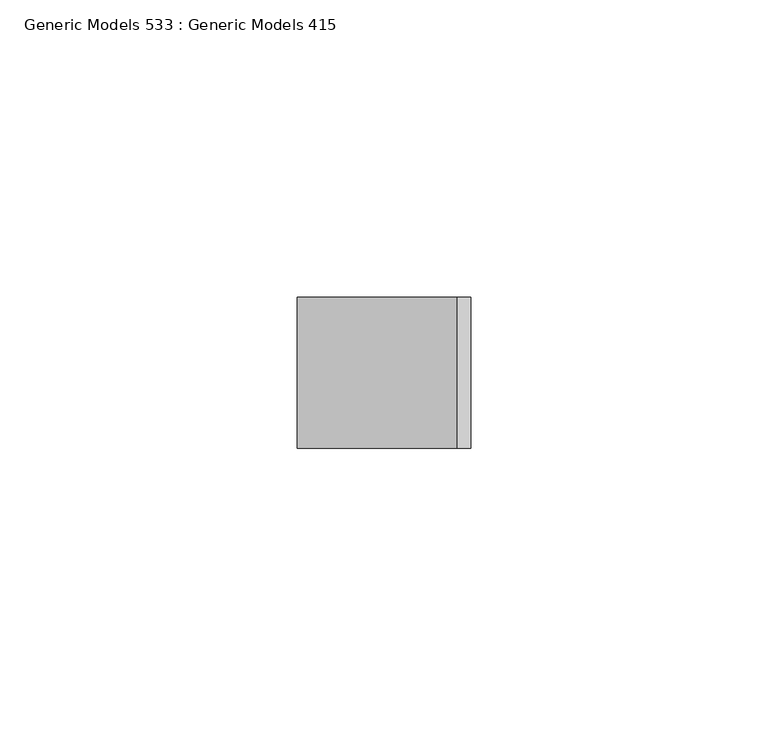
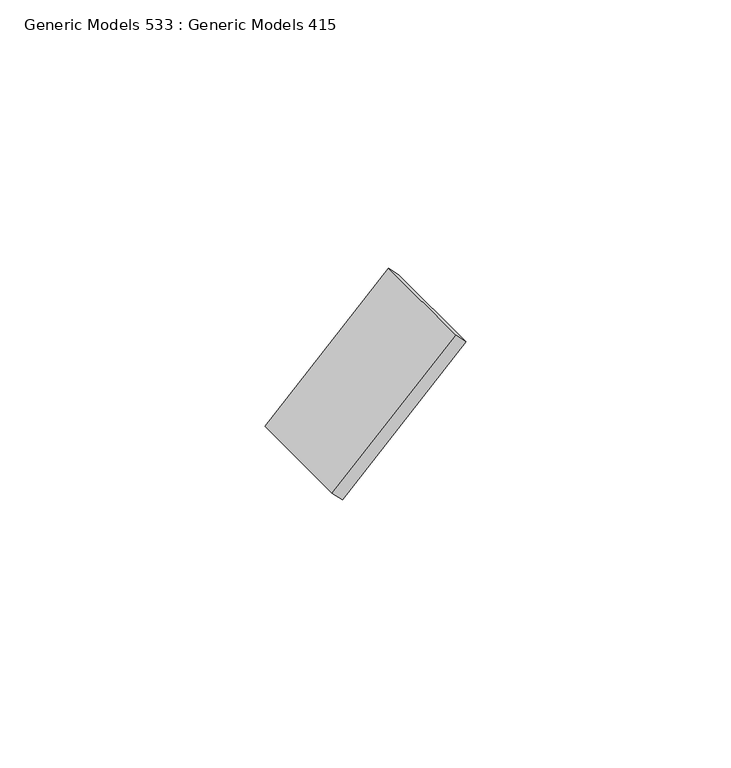
"""IFC4 building model written with IfcOpenShell, lengths in millimetres: proxy geometry, Generic Models 533 : Generic Models 415."""

import ifcopenshell
import ifcopenshell.guid

model = None  # the IFC model being written
_history = None  # IfcOwnerHistory: only IFC2X3 demands one
_inside = {}  # id of a spatial element -> (the spatial element, [elements in it])
_under = {}  # id of a project, library or spatial element -> (it, [spatial elements below it])
_declared = {}  # id of a project -> (the project, [libraries it declares])
_typed = {}  # id of a type object -> (the type object, [elements of that type])
_made_of = {}  # id of a material, layer set ... -> (it, [elements and type objects made of it])


def new_model(schema):
    """Start an empty IFC model of exactly this schema.

    Asked for "IFC4X3", IfcOpenShell would pick the latest addendum, in which some entities
    have other attributes; the version numbers below select the first issue.
    IFC2X3 requires an IfcOwnerHistory on every rooted entity: one is made here for all.
    """
    global model, _history
    if schema == "IFC4X3":
        model = ifcopenshell.file(schema_version=(4, 3, 0, 0))
    else:
        model = ifcopenshell.file(schema=schema)
    _inside.clear()
    _under.clear()
    _declared.clear()
    _typed.clear()
    _made_of.clear()
    _history = None
    if model.schema == "IFC2X3":
        org = make("IfcOrganization", Name="unknown")
        user = make(
            "IfcPersonAndOrganization",
            ThePerson=make("IfcPerson", FamilyName="unknown"),
            TheOrganization=org,
        )
        app = make(
            "IfcApplication",
            ApplicationDeveloper=org,
            Version="unknown",
            ApplicationFullName="unknown",
            ApplicationIdentifier="unknown",
        )
        _history = make(
            "IfcOwnerHistory",
            OwningUser=user,
            OwningApplication=app,
            ChangeAction="ADDED",
            CreationDate=0,
        )
    return model


def make(cls, **values):
    """One entity of the class cls with the attributes given. An attribute that is None is left unset."""
    return model.create_entity(
        cls, **{name: value for name, value in values.items() if value is not None}
    )


def rooted(cls, **values):
    """An entity with a GlobalId (a new one), such as an element, a storey or a relation."""
    return make(cls, GlobalId=ifcopenshell.guid.new(), OwnerHistory=_history, **values)


def si_unit(unit_type, name, prefix=None):
    """IfcSIUnit, for example si_unit("LENGTHUNIT", "METRE", prefix="MILLI")."""
    return make("IfcSIUnit", UnitType=unit_type, Prefix=prefix, Name=name)


def assignment(units):
    """IfcUnitAssignment: the units of a project."""
    return None if units is None else make("IfcUnitAssignment", Units=units)


def point(xyz):
    """IfcCartesianPoint."""
    return None if xyz is None else make("IfcCartesianPoint", Coordinates=xyz)


def direction(xyz):
    """IfcDirection."""
    return None if xyz is None else make("IfcDirection", DirectionRatios=xyz)


def frame(location, z_axis=None, x_axis=None):
    """IfcAxis2Placement3D, a coordinate frame: its origin and axes. An axis left out is left unset."""
    return make(
        "IfcAxis2Placement3D",
        Location=point(location),
        Axis=direction(z_axis),
        RefDirection=direction(x_axis),
    )


def origin():
    """The frame at (0, 0, 0) with its axes left unset."""
    return frame((0.0, 0.0, 0.0))


def place(relative_to, where):
    """IfcLocalPlacement: puts the frame where relative to a parent placement (None: the world)."""
    return make(
        "IfcLocalPlacement", PlacementRelTo=relative_to, RelativePlacement=where
    )


def context(
    kind, dimensions, precision=None, world=None, true_north=None, identifier=None
):
    """IfcGeometricRepresentationContext, for example the 3D "Model" context."""
    return make(
        "IfcGeometricRepresentationContext",
        ContextIdentifier=identifier,
        ContextType=kind,
        CoordinateSpaceDimension=dimensions,
        Precision=precision,
        WorldCoordinateSystem=world,
        TrueNorth=true_north,
    )


def project(units=None, contexts=None):
    """IfcProject with its units and contexts."""
    return rooted(
        "IfcProject",
        Name="project",
        RepresentationContexts=contexts,
        UnitsInContext=assignment(units),
    )


def spatial(cls, under=None, at=None, **own):
    """A site, building, storey or space (cls), placed at a placement, below another one or the project."""
    s = rooted(cls, ObjectPlacement=at, **own)
    if under is not None:
        _under.setdefault(under.id(), (under, []))[1].append(s)
    return s


def polyline(points):
    """IfcPolyline through the points."""
    return make("IfcPolyline", Points=[point(p) for p in points])


def outline(outer, holes=None, kind="AREA"):
    """IfcArbitraryClosedProfileDef: a profile drawn as a closed curve; with holes, ...WithVoids."""
    if holes is None:
        return make("IfcArbitraryClosedProfileDef", ProfileType=kind, OuterCurve=outer)
    return make(
        "IfcArbitraryProfileDefWithVoids",
        ProfileType=kind,
        OuterCurve=outer,
        InnerCurves=holes,
    )


def extrude(swept, where, along, depth):
    """IfcExtrudedAreaSolid: the profile swept, set in the frame where, extruded along a direction by depth."""
    return make(
        "IfcExtrudedAreaSolid",
        SweptArea=swept,
        Position=where,
        ExtrudedDirection=direction(along),
        Depth=depth,
    )


def shape(context_of_items, identifier, shape_type, items):
    """IfcShapeRepresentation: the items that make up one representation, for example the "Body"."""
    return make(
        "IfcShapeRepresentation",
        ContextOfItems=context_of_items,
        RepresentationIdentifier=identifier,
        RepresentationType=shape_type,
        Items=items,
    )


def source(mapping_origin, context_of_items, identifier, shape_type, items):
    """IfcRepresentationMap: a shape defined once, which mapped items show again and again."""
    return make(
        "IfcRepresentationMap",
        MappingOrigin=mapping_origin,
        MappedRepresentation=shape(context_of_items, identifier, shape_type, items),
    )


def transform(
    local_origin,
    x_axis=None,
    y_axis=None,
    z_axis=None,
    scale=None,
    scale2=None,
    scale3=None,
    uniform=True,
):
    """IfcCartesianTransformationOperator3D, or its non-uniform kind. x_axis, y_axis, z_axis: its Axis1, 2, 3."""
    if uniform:
        return make(
            "IfcCartesianTransformationOperator3D",
            Axis1=direction(x_axis),
            Axis2=direction(y_axis),
            LocalOrigin=point(local_origin),
            Scale=scale,
            Axis3=direction(z_axis),
        )
    return make(
        "IfcCartesianTransformationOperator3DnonUniform",
        Axis1=direction(x_axis),
        Axis2=direction(y_axis),
        LocalOrigin=point(local_origin),
        Scale=scale,
        Axis3=direction(z_axis),
        Scale2=scale2,
        Scale3=scale3,
    )


def mapped(mapping_source, mapping_target):
    """IfcMappedItem: shows the shape of a source again, moved by a transform."""
    return make(
        "IfcMappedItem", MappingSource=mapping_source, MappingTarget=mapping_target
    )


def made_of(thing, what):
    """Note that an element or type object is made of a material, layer set ...; save() writes the relation."""
    if what is not None:
        _made_of.setdefault(what.id(), (what, []))[1].append(thing)
    return thing


def element(
    cls,
    number,
    at=None,
    inside=None,
    cuts=None,
    type_object=None,
    material=None,
    context=None,
    identifier="Body",
    shape_type=None,
    held_by="IfcProductDefinitionShape",
    body=None,
    shapes=None,
    **own,
):
    """One element of the class cls, such as IfcWall. Its Tag is "e" and its number.

    at: its placement. inside: the storey or other place that contains it. cuts: it is an
    opening in that element (IfcRelVoidsElement). A single representation is given by context,
    identifier, shape_type and body (its items); several are given by shapes. held_by: the class
    of the entity that holds the representations. save() writes the other relations.
    """
    e = rooted(cls, Tag="e%d" % number, ObjectPlacement=at, **own)
    if body is not None:
        shapes = [shape(context, identifier, shape_type, body)]
    if shapes is not None:
        e.Representation = make(held_by, Representations=shapes)
    if inside is not None:
        _inside.setdefault(inside.id(), (inside, []))[1].append(e)
    if cuts is not None:
        rooted(
            "IfcRelVoidsElement", RelatingBuildingElement=cuts, RelatedOpeningElement=e
        )
    if type_object is not None:
        _typed.setdefault(type_object.id(), (type_object, []))[1].append(e)
    return made_of(e, material)


def aggregate(whole, parts):
    """IfcRelAggregates: a whole, such as a stair, and the parts it consists of."""
    return rooted("IfcRelAggregates", RelatingObject=whole, RelatedObjects=parts)


def save(model, path):
    """Write the relations noted so far, then the file.

    IfcRelAggregates (storeys below a building ...), IfcRelContainedInSpatialStructure (elements
    in a storey), IfcRelDefinesByType, IfcRelAssociatesMaterial and IfcRelDeclares: one each for
    every whole, place, type object, material and project.
    """
    for whole, parts in _under.values():
        aggregate(whole, parts)
    for where, things in _inside.values():
        rooted(
            "IfcRelContainedInSpatialStructure",
            RelatedElements=things,
            RelatingStructure=where,
        )
    for kind, things in _typed.values():
        rooted("IfcRelDefinesByType", RelatedObjects=things, RelatingType=kind)
    for what, things in _made_of.values():
        rooted("IfcRelAssociatesMaterial", RelatedObjects=things, RelatingMaterial=what)
    for by, libraries in _declared.values():
        rooted("IfcRelDeclares", RelatingContext=by, RelatedDefinitions=libraries)
    model.write(path)


def generic_models_533_generic_models_415_e4f0f834(model_context):
    return source(origin(), model_context, "Body", "SweptSolid", [
        extrude(outline(polyline([(0.0, -3.175), (0.0, 0.0), (25.4, 0.0), (25.4, -3.175), (0.0, -3.175)])), frame((7848.0411784, 4501.3863946, 125257.8849742), z_axis=(0.7071067811867181, 0.0, 0.707106781186377), x_axis=(0.0, -1.0, 0.0)), (0.0, 0.0, 1.0), 38.1),
    ])


if __name__ == "__main__":
    model = new_model("IFC4")
    model_context = context("Model", 3, world=origin())
    ifc_project = project(units=[si_unit("LENGTHUNIT", "METRE", prefix="MILLI")], contexts=[model_context])
    site = spatial("IfcSite", under=ifc_project)
    building = spatial("IfcBuilding", under=site)
    placement = place(None, origin())
    generic_models_533_generic_models_415_shape = generic_models_533_generic_models_415_e4f0f834(model_context)
    element("IfcBuildingElementProxy", 1, Name="Generic Models 533 : Generic Models 415", ObjectType="Generic Models 533 : Generic Models 415", at=placement, inside=building, context=model_context, shape_type="MappedRepresentation", body=[
        mapped(generic_models_533_generic_models_415_shape, transform((0.0, 0.0, 0.0), x_axis=(1.0, 0.0, 0.0), y_axis=(0.0, 1.0, 0.0), z_axis=(0.0, 0.0, 1.0))),
    ])
    save(model, "model.ifc")

# Revit data of these elements
# Element 1 (IfcBuildingElementProxy, "Generic Models 533 : Generic Models 415")
#   Materials on its faces: "_WELDED STEEL TABS FOR LOUVER ATTACHMENT"
# Materials
#   "_WELDED STEEL TABS FOR LOUVER ATTACHMENT": class "Metal", colour RGB 199 199 199, transparency 0, Description = "Structural steel 50ksi", Cost = 0
